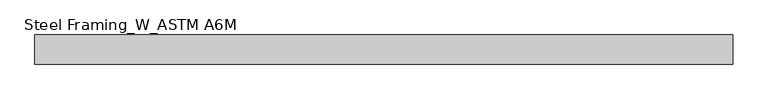
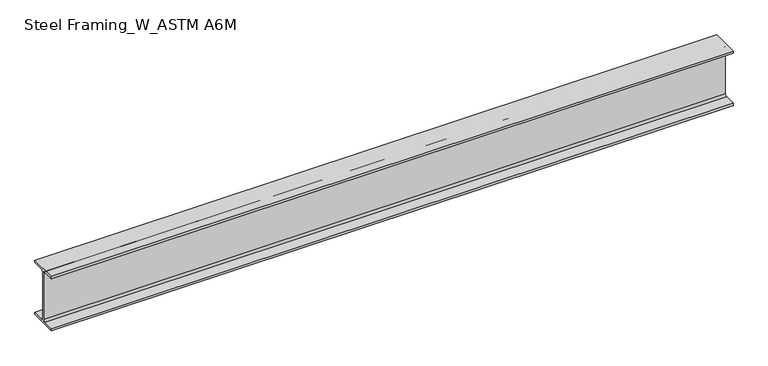
"""IFC4 building model written with IfcOpenShell, lengths in millimetres: beam geometry, Steel Framing_W_ASTM A6M : H_SB_AR_S02_W200x22.5_J1."""

from ifc_helpers import new_model, si_unit, point, frame, frame_2d, origin, place, context, project, spatial, polyline, circle_curve, trimmed, segment, composite_curve, outline, extrude, source, transform, mapped, element, save


def steel_framing_w_astm_a6m_45b14fa7(model_context):
    return source(origin(), model_context, "Body", "SweptSolid", [
        extrude(outline(composite_curve([segment(polyline([(51.0, -95.0), (51.0, -103.0), (-51.0, -103.0), (-51.0, -95.0), (-10.71, -95.0)]), True, "CONTINUOUS"), segment(trimmed(circle_curve(frame_2d((-10.71, -87.4)), 7.6), [point((-10.71, -95.0))], [point((-3.11, -87.4))], True, "CARTESIAN"), True, "CONTINUOUS"), segment(polyline([(-3.11, -87.4), (-3.11, 87.4)]), True, "CONTINUOUS"), segment(trimmed(circle_curve(frame_2d((-10.71, 87.4)), 7.6), [point((-3.11, 87.4))], [point((-10.71, 95.0))], True, "CARTESIAN"), True, "CONTINUOUS"), segment(polyline([(-10.71, 95.0), (-51.0, 95.0), (-51.0, 103.0), (51.0, 103.0), (51.0, 95.0), (10.71, 95.0)]), True, "CONTINUOUS"), segment(trimmed(circle_curve(frame_2d((10.71, 87.4)), 7.6), [point((10.71, 95.0))], [point((3.11, 87.4))], True, "CARTESIAN"), True, "CONTINUOUS"), segment(polyline([(3.11, 87.4), (3.11, -87.4)]), True, "CONTINUOUS"), segment(trimmed(circle_curve(frame_2d((10.71, -87.4)), 7.6), [point((3.11, -87.4))], [point((10.71, -95.0))], True, "CARTESIAN"), True, "CONTINUOUS"), segment(polyline([(10.71, -95.0), (51.0, -95.0)]), True, "CONTINUOUS")], self_intersect=False)), frame((-1192.8, 0.0, 0.0), z_axis=(1.0, 0.0, 0.0), x_axis=(0.0, 1.0, 0.0)), (0.0, 0.0, 1.0), 2445.6),
    ])


if __name__ == "__main__":
    model = new_model("IFC4")
    model_context = context("Model", 3, world=origin())
    ifc_project = project(units=[si_unit("LENGTHUNIT", "METRE", prefix="MILLI")], contexts=[model_context])
    site = spatial("IfcSite", under=ifc_project)
    building = spatial("IfcBuilding", under=site)
    placement = place(None, origin())
    steel_framing_w_astm_a6m_shape = steel_framing_w_astm_a6m_45b14fa7(model_context)
    element("IfcBeam", 1, ObjectType="Steel Framing_W_ASTM A6M : H_SB_AR_S02_W200x22.5_J1", at=placement, inside=building, context=model_context, shape_type="MappedRepresentation", body=[
        mapped(steel_framing_w_astm_a6m_shape, transform((0.0, 0.0, 0.0), x_axis=(1.0, 0.0, 0.0), y_axis=(0.0, 1.0, 0.0), z_axis=(0.0, 0.0, 1.0))),
    ])
    save(model, "model.ifc")

# Revit data of these elements
# Type "Steel Framing_W_ASTM A6M : H_SB_AR_S02_W200x22.5_J1"
#   Section Name Key = "W8x15"
#   Width = 10.2 cm
#   Web Thickness = 0.622 cm
#   Web Fillet = 0.76 cm
#   Warping Constant = 13900.0 cm⁶
#   Torsional Moment of Inertia = 5.70 cm⁴
#   Section Area = 28.6 cm²
#   Plastic Modulus weak axis = 43.8 cm³
#   Plastic Modulus strong axis = 223.0 cm³
#   Perimeter = 0.795 m²/m
#   Nominal Weight = 22.50 kgf/m
#   Moment of Inertia weak axis = 142.00 cm⁴
#   Moment of Inertia strong axis = 2000.00 cm⁴
#   Height = 20.6 cm
#   Flange Thickness = 0.8 cm
#   Elastic Modulus weak axis = 27.9 cm³
#   Elastic Modulus strong axis = 193.0 cm³
#   Centroid Vertical = 10.3 cm
#   Centroid Horizontal = 5.1 cm
#   Length [instance default] = 1500 mm
#   Structural Material [instance default] = Steel, 45-345
#   Bolt Spacing = 0
#   Assembly Code = ""
# Element 1 (IfcBeam, "Steel Framing_W_ASTM A6M : H_SB_AR_S02_W200x22.5_J1")
#   Materials on its faces: "Steel, 45-345"
# Materials
#   "Steel, 45-345": class "Metal", colour RGB 189 187 185, transparency 0, Description = "Steel 345 MPa", Cost = 0
